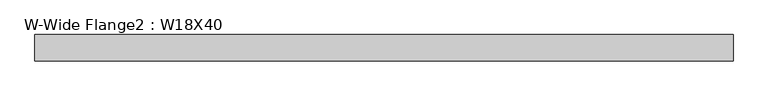
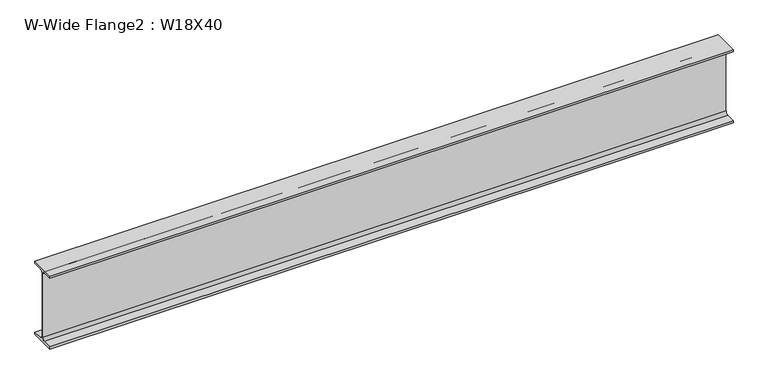
"""IFC4 building model written with IfcOpenShell, lengths in millimetres: beam geometry, W-Wide Flange2 : W18X40."""

from ifc_helpers import new_model, si_unit, point, frame, frame_2d, origin, place, context, project, spatial, polyline, circle_curve, trimmed, segment, composite_curve, outline, extrude, source, transform, mapped, element, save


def w_wide_flange2_w18x40_962a7e4b(model_context):
    return source(origin(), model_context, "Body", "SweptSolid", [
        extrude(outline(composite_curve([segment(polyline([(76.454, -213.995), (76.454, -227.33), (-76.454, -227.33), (-76.454, -213.995), (-20.828, -213.995)]), True, "CONTINUOUS"), segment(trimmed(circle_curve(frame_2d((-20.828, -197.1675)), 16.8275), [point((-20.828, -213.995))], [point((-4.0005, -197.1675))], True, "CARTESIAN"), True, "CONTINUOUS"), segment(polyline([(-4.0005, -197.1675), (-4.0005, 197.1675)]), True, "CONTINUOUS"), segment(trimmed(circle_curve(frame_2d((-20.828, 197.1675)), 16.8275), [point((-4.0005, 197.1675))], [point((-20.828, 213.995))], True, "CARTESIAN"), True, "CONTINUOUS"), segment(polyline([(-20.828, 213.995), (-76.454, 213.995), (-76.454, 227.33), (76.454, 227.33), (76.454, 213.995), (20.828, 213.995)]), True, "CONTINUOUS"), segment(trimmed(circle_curve(frame_2d((20.828, 197.1675)), 16.8275), [point((20.828, 213.995))], [point((4.0005, 197.1675))], True, "CARTESIAN"), True, "CONTINUOUS"), segment(polyline([(4.0005, 197.1675), (4.0005, -197.1675)]), True, "CONTINUOUS"), segment(trimmed(circle_curve(frame_2d((20.828, -197.1675)), 16.8275), [point((4.0005, -197.1675))], [point((20.828, -213.995))], True, "CARTESIAN"), True, "CONTINUOUS"), segment(polyline([(20.828, -213.995), (76.454, -213.995)]), True, "CONTINUOUS")], self_intersect=False)), frame((-2012.553125, 0.0, 0.0), z_axis=(1.0, 0.0, 0.0), x_axis=(0.0, 1.0, 0.0)), (0.0, 0.0, 1.0), 4025.10625),
    ])


if __name__ == "__main__":
    model = new_model("IFC4")
    model_context = context("Model", 3, world=origin())
    ifc_project = project(units=[si_unit("LENGTHUNIT", "METRE", prefix="MILLI")], contexts=[model_context])
    site = spatial("IfcSite", under=ifc_project)
    building = spatial("IfcBuilding", under=site)
    placement = place(None, origin())
    w_wide_flange2_w18x40_shape = w_wide_flange2_w18x40_962a7e4b(model_context)
    element("IfcBeam", 1, ObjectType="W-Wide Flange2 : W18X40", at=placement, inside=building, context=model_context, shape_type="MappedRepresentation", body=[
        mapped(w_wide_flange2_w18x40_shape, transform((0.0, 0.0, 0.0), x_axis=(1.0, 0.0, 0.0), y_axis=(0.0, 1.0, 0.0), z_axis=(0.0, 0.0, 1.0))),
    ])
    save(model, "model.ifc")

# Revit data of these elements
# Type "W-Wide Flange2 : W18X40"
#   Assembly Code = "B10"
#   W = 40
#   Length [instance default] = 5' - 0"
#   bf = 0' - 6.02"
#   d = 1' - 5.9"
#   k = 0' - 1 3/16"
#   k2 = 0' - 0.6625"
#   tf = 0' - 0.525"
#   tw = 0' - 0.315"
#   A = 0.0819444 SF
#   Structural Material [instance default] = Steel ASTM A992
# Element 1 (IfcBeam, "W-Wide Flange2 : W18X40")
#   Materials on its faces: "Steel ASTM A992"
# Materials
#   "Steel ASTM A992": class "Metal", colour RGB 199 199 199, transparency 0, Description = "Structural steel 50ksi", Cost = 0
